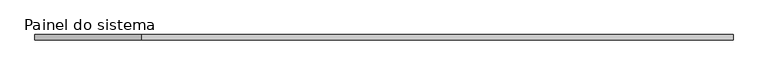
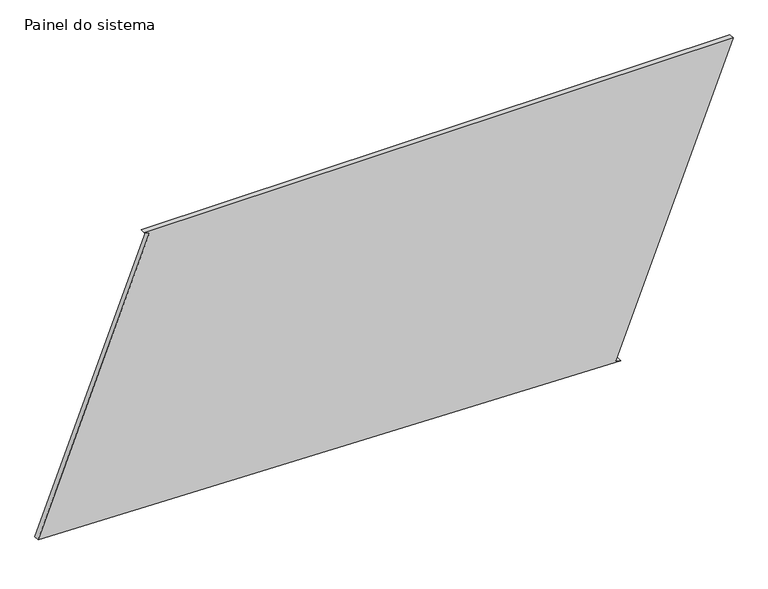
"""IFC4 building model written with IfcOpenShell, lengths in millimetres: plate geometry, Painel do sistema : Envidraçado."""

from ifc_helpers import new_model, si_unit, frame, origin, place, context, project, spatial, polyline, outline, extrude, source, transform, mapped, element, save


def painel_do_sistema_2d5f6f3b(model_context):
    return source(origin(), model_context, "Body", "SweptSolid", [
        extrude(outline(polyline([(0.0, 1093.5357577), (9.0972802, 1070.2497213), (1403.0263917, 1614.8234539), (1403.0263917, -1120.323151), (1393.9291114, -1097.0371146), (68.5668902, -1614.8234539), (0.0, 1093.5357577)])), frame((0.0, 24.5, 0.0), z_axis=(0.0, 1.0, 0.0), x_axis=(0.0, 0.0, 1.0)), (0.0, 0.0, 1.0), 25.0),
    ])


if __name__ == "__main__":
    model = new_model("IFC4")
    model_context = context("Model", 3, world=origin())
    ifc_project = project(units=[si_unit("LENGTHUNIT", "METRE", prefix="MILLI")], contexts=[model_context])
    site = spatial("IfcSite", under=ifc_project)
    building = spatial("IfcBuilding", under=site)
    placement = place(None, origin())
    painel_do_sistema_shape = painel_do_sistema_2d5f6f3b(model_context)
    element("IfcPlate", 1, ObjectType="Painel do sistema : Envidraçado", at=placement, inside=building, context=model_context, shape_type="MappedRepresentation", body=[
        mapped(painel_do_sistema_shape, transform((0.0, 0.0, 0.0), x_axis=(1.0, 0.0, 0.0), y_axis=(0.0, 1.0, 0.0), z_axis=(0.0, 0.0, 1.0))),
    ])
    save(model, "model.ifc")

# Revit data of these elements
# Type "Painel do sistema : Envidraçado"
#   Construction Type Id = "GSP4R"
#   Analytic Construction = "Vidraça única Pilkington 1/8 pol"
#   Visual Light Transmittance = 0.9
#   Solar Heat Gain Coefficient = 0.86
#   Heat Transfer Coefficient (U) = 6.7069 W/(m²·K)
# Element 1 (IfcPlate, "Painel do sistema : Envidraçado")
#   Materials on its faces: "Vidro"
# Materials
#   "Vidro": class "Vidro", colour RGB 0 128 192, transparency 0.9, Description = "Vidro de sílica", Cost = 0
